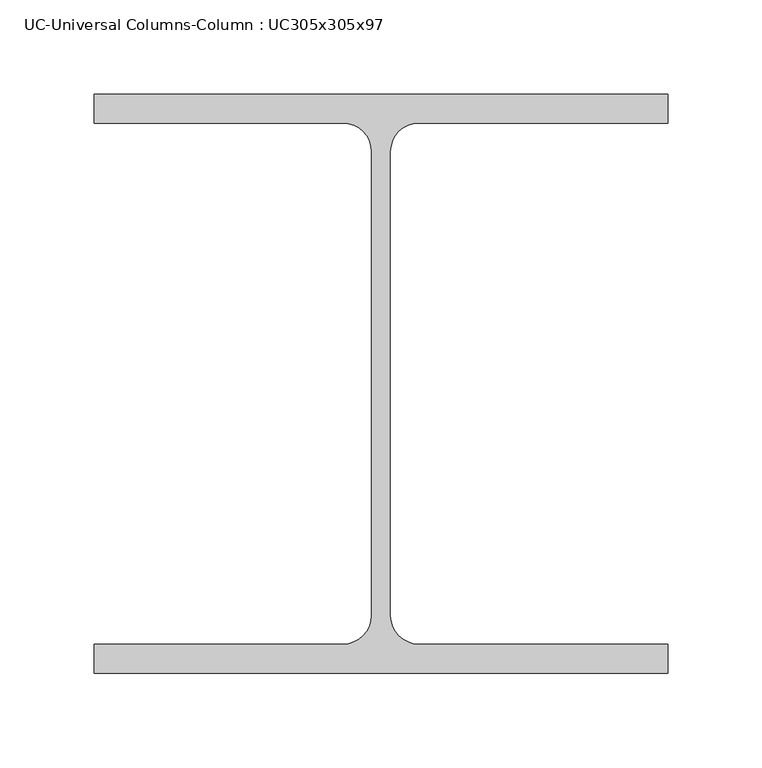
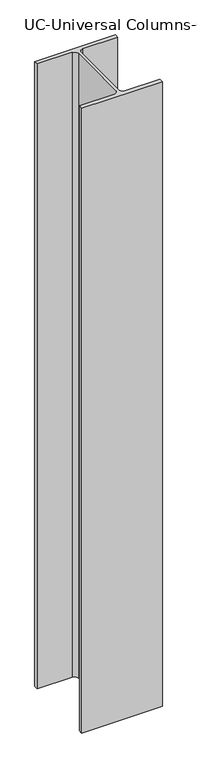
"""IFC4 building model written with IfcOpenShell, lengths in millimetres: column geometry, UC-Universal Columns-Column : UC305x305x97."""

import ifcopenshell
import ifcopenshell.guid

model = None  # the IFC model being written
_history = None  # IfcOwnerHistory: only IFC2X3 demands one
_inside = {}  # id of a spatial element -> (the spatial element, [elements in it])
_under = {}  # id of a project, library or spatial element -> (it, [spatial elements below it])
_declared = {}  # id of a project -> (the project, [libraries it declares])
_typed = {}  # id of a type object -> (the type object, [elements of that type])
_made_of = {}  # id of a material, layer set ... -> (it, [elements and type objects made of it])


def new_model(schema):
    """Start an empty IFC model of exactly this schema.

    Asked for "IFC4X3", IfcOpenShell would pick the latest addendum, in which some entities
    have other attributes; the version numbers below select the first issue.
    IFC2X3 requires an IfcOwnerHistory on every rooted entity: one is made here for all.
    """
    global model, _history
    if schema == "IFC4X3":
        model = ifcopenshell.file(schema_version=(4, 3, 0, 0))
    else:
        model = ifcopenshell.file(schema=schema)
    _inside.clear()
    _under.clear()
    _declared.clear()
    _typed.clear()
    _made_of.clear()
    _history = None
    if model.schema == "IFC2X3":
        org = make("IfcOrganization", Name="unknown")
        user = make(
            "IfcPersonAndOrganization",
            ThePerson=make("IfcPerson", FamilyName="unknown"),
            TheOrganization=org,
        )
        app = make(
            "IfcApplication",
            ApplicationDeveloper=org,
            Version="unknown",
            ApplicationFullName="unknown",
            ApplicationIdentifier="unknown",
        )
        _history = make(
            "IfcOwnerHistory",
            OwningUser=user,
            OwningApplication=app,
            ChangeAction="ADDED",
            CreationDate=0,
        )
    return model


def make(cls, **values):
    """One entity of the class cls with the attributes given. An attribute that is None is left unset."""
    return model.create_entity(
        cls, **{name: value for name, value in values.items() if value is not None}
    )


def rooted(cls, **values):
    """An entity with a GlobalId (a new one), such as an element, a storey or a relation."""
    return make(cls, GlobalId=ifcopenshell.guid.new(), OwnerHistory=_history, **values)


def si_unit(unit_type, name, prefix=None):
    """IfcSIUnit, for example si_unit("LENGTHUNIT", "METRE", prefix="MILLI")."""
    return make("IfcSIUnit", UnitType=unit_type, Prefix=prefix, Name=name)


def assignment(units):
    """IfcUnitAssignment: the units of a project."""
    return None if units is None else make("IfcUnitAssignment", Units=units)


def point(xyz):
    """IfcCartesianPoint."""
    return None if xyz is None else make("IfcCartesianPoint", Coordinates=xyz)


def direction(xyz):
    """IfcDirection."""
    return None if xyz is None else make("IfcDirection", DirectionRatios=xyz)


def frame(location, z_axis=None, x_axis=None):
    """IfcAxis2Placement3D, a coordinate frame: its origin and axes. An axis left out is left unset."""
    return make(
        "IfcAxis2Placement3D",
        Location=point(location),
        Axis=direction(z_axis),
        RefDirection=direction(x_axis),
    )


def frame_2d(location, x_axis=None):
    """IfcAxis2Placement2D, a coordinate frame in the plane: its origin and x axis."""
    return make(
        "IfcAxis2Placement2D", Location=point(location), RefDirection=direction(x_axis)
    )


def origin():
    """The frame at (0, 0, 0) with its axes left unset."""
    return frame((0.0, 0.0, 0.0))


def origin_with_axes():
    """The frame at (0, 0, 0) with the z axis (0, 0, 1) and the x axis (1, 0, 0) written out."""
    return frame((0.0, 0.0, 0.0), z_axis=(0.0, 0.0, 1.0), x_axis=(1.0, 0.0, 0.0))


def place(relative_to, where):
    """IfcLocalPlacement: puts the frame where relative to a parent placement (None: the world)."""
    return make(
        "IfcLocalPlacement", PlacementRelTo=relative_to, RelativePlacement=where
    )


def context(
    kind, dimensions, precision=None, world=None, true_north=None, identifier=None
):
    """IfcGeometricRepresentationContext, for example the 3D "Model" context."""
    return make(
        "IfcGeometricRepresentationContext",
        ContextIdentifier=identifier,
        ContextType=kind,
        CoordinateSpaceDimension=dimensions,
        Precision=precision,
        WorldCoordinateSystem=world,
        TrueNorth=true_north,
    )


def project(units=None, contexts=None):
    """IfcProject with its units and contexts."""
    return rooted(
        "IfcProject",
        Name="project",
        RepresentationContexts=contexts,
        UnitsInContext=assignment(units),
    )


def spatial(cls, under=None, at=None, **own):
    """A site, building, storey or space (cls), placed at a placement, below another one or the project."""
    s = rooted(cls, ObjectPlacement=at, **own)
    if under is not None:
        _under.setdefault(under.id(), (under, []))[1].append(s)
    return s


def polyline(points):
    """IfcPolyline through the points."""
    return make("IfcPolyline", Points=[point(p) for p in points])


def circle_curve(where, radius):
    """IfcCircle in the frame where."""
    return make("IfcCircle", Position=where, Radius=radius)


def trimmed(basis, trim1, trim2, sense, master):
    """IfcTrimmedCurve: the piece of a basis curve between two trims."""
    return make(
        "IfcTrimmedCurve",
        BasisCurve=basis,
        Trim1=trim1,
        Trim2=trim2,
        SenseAgreement=sense,
        MasterRepresentation=master,
    )


def segment(curve, same_sense, transition):
    """IfcCompositeCurveSegment."""
    return make(
        "IfcCompositeCurveSegment",
        Transition=transition,
        SameSense=same_sense,
        ParentCurve=curve,
    )


def composite_curve(segments, self_intersect=None):
    """IfcCompositeCurve: segments joined end to end."""
    return make("IfcCompositeCurve", Segments=segments, SelfIntersect=self_intersect)


def outline(outer, holes=None, kind="AREA"):
    """IfcArbitraryClosedProfileDef: a profile drawn as a closed curve; with holes, ...WithVoids."""
    if holes is None:
        return make("IfcArbitraryClosedProfileDef", ProfileType=kind, OuterCurve=outer)
    return make(
        "IfcArbitraryProfileDefWithVoids",
        ProfileType=kind,
        OuterCurve=outer,
        InnerCurves=holes,
    )


def extrude(swept, where, along, depth):
    """IfcExtrudedAreaSolid: the profile swept, set in the frame where, extruded along a direction by depth."""
    return make(
        "IfcExtrudedAreaSolid",
        SweptArea=swept,
        Position=where,
        ExtrudedDirection=direction(along),
        Depth=depth,
    )


def shape(context_of_items, identifier, shape_type, items):
    """IfcShapeRepresentation: the items that make up one representation, for example the "Body"."""
    return make(
        "IfcShapeRepresentation",
        ContextOfItems=context_of_items,
        RepresentationIdentifier=identifier,
        RepresentationType=shape_type,
        Items=items,
    )


def source(mapping_origin, context_of_items, identifier, shape_type, items):
    """IfcRepresentationMap: a shape defined once, which mapped items show again and again."""
    return make(
        "IfcRepresentationMap",
        MappingOrigin=mapping_origin,
        MappedRepresentation=shape(context_of_items, identifier, shape_type, items),
    )


def transform(
    local_origin,
    x_axis=None,
    y_axis=None,
    z_axis=None,
    scale=None,
    scale2=None,
    scale3=None,
    uniform=True,
):
    """IfcCartesianTransformationOperator3D, or its non-uniform kind. x_axis, y_axis, z_axis: its Axis1, 2, 3."""
    if uniform:
        return make(
            "IfcCartesianTransformationOperator3D",
            Axis1=direction(x_axis),
            Axis2=direction(y_axis),
            LocalOrigin=point(local_origin),
            Scale=scale,
            Axis3=direction(z_axis),
        )
    return make(
        "IfcCartesianTransformationOperator3DnonUniform",
        Axis1=direction(x_axis),
        Axis2=direction(y_axis),
        LocalOrigin=point(local_origin),
        Scale=scale,
        Axis3=direction(z_axis),
        Scale2=scale2,
        Scale3=scale3,
    )


def mapped(mapping_source, mapping_target):
    """IfcMappedItem: shows the shape of a source again, moved by a transform."""
    return make(
        "IfcMappedItem", MappingSource=mapping_source, MappingTarget=mapping_target
    )


def made_of(thing, what):
    """Note that an element or type object is made of a material, layer set ...; save() writes the relation."""
    if what is not None:
        _made_of.setdefault(what.id(), (what, []))[1].append(thing)
    return thing


def element(
    cls,
    number,
    at=None,
    inside=None,
    cuts=None,
    type_object=None,
    material=None,
    context=None,
    identifier="Body",
    shape_type=None,
    held_by="IfcProductDefinitionShape",
    body=None,
    shapes=None,
    **own,
):
    """One element of the class cls, such as IfcWall. Its Tag is "e" and its number.

    at: its placement. inside: the storey or other place that contains it. cuts: it is an
    opening in that element (IfcRelVoidsElement). A single representation is given by context,
    identifier, shape_type and body (its items); several are given by shapes. held_by: the class
    of the entity that holds the representations. save() writes the other relations.
    """
    e = rooted(cls, Tag="e%d" % number, ObjectPlacement=at, **own)
    if body is not None:
        shapes = [shape(context, identifier, shape_type, body)]
    if shapes is not None:
        e.Representation = make(held_by, Representations=shapes)
    if inside is not None:
        _inside.setdefault(inside.id(), (inside, []))[1].append(e)
    if cuts is not None:
        rooted(
            "IfcRelVoidsElement", RelatingBuildingElement=cuts, RelatedOpeningElement=e
        )
    if type_object is not None:
        _typed.setdefault(type_object.id(), (type_object, []))[1].append(e)
    return made_of(e, material)


def aggregate(whole, parts):
    """IfcRelAggregates: a whole, such as a stair, and the parts it consists of."""
    return rooted("IfcRelAggregates", RelatingObject=whole, RelatedObjects=parts)


def save(model, path):
    """Write the relations noted so far, then the file.

    IfcRelAggregates (storeys below a building ...), IfcRelContainedInSpatialStructure (elements
    in a storey), IfcRelDefinesByType, IfcRelAssociatesMaterial and IfcRelDeclares: one each for
    every whole, place, type object, material and project.
    """
    for whole, parts in _under.values():
        aggregate(whole, parts)
    for where, things in _inside.values():
        rooted(
            "IfcRelContainedInSpatialStructure",
            RelatedElements=things,
            RelatingStructure=where,
        )
    for kind, things in _typed.values():
        rooted("IfcRelDefinesByType", RelatedObjects=things, RelatingType=kind)
    for what, things in _made_of.values():
        rooted("IfcRelAssociatesMaterial", RelatedObjects=things, RelatingMaterial=what)
    for by, libraries in _declared.values():
        rooted("IfcRelDeclares", RelatingContext=by, RelatedDefinitions=libraries)
    model.write(path)


def uc_universal_columns_column_uc305x305x97_3ae92ab7(model_context):
    return source(origin(), model_context, "Body", "SweptSolid", [
        extrude(outline(composite_curve([segment(polyline([(152.65, 153.95), (152.65, 138.55), (20.15, 138.55)]), True, "CONTINUOUS"), segment(trimmed(circle_curve(frame_2d((20.15, 123.35)), 15.2), [point((20.15, 138.55))], [point((4.95, 123.35))], True, "CARTESIAN"), True, "CONTINUOUS"), segment(polyline([(4.95, 123.35), (4.95, -123.35)]), True, "CONTINUOUS"), segment(trimmed(circle_curve(frame_2d((20.15, -123.35)), 15.2), [point((4.95, -123.35))], [point((20.15, -138.55))], True, "CARTESIAN"), True, "CONTINUOUS"), segment(polyline([(20.15, -138.55), (152.65, -138.55), (152.65, -153.95), (-152.65, -153.95), (-152.65, -138.55), (-20.15, -138.55)]), True, "CONTINUOUS"), segment(trimmed(circle_curve(frame_2d((-20.15, -123.35)), 15.2), [point((-20.15, -138.55))], [point((-4.95, -123.35))], True, "CARTESIAN"), True, "CONTINUOUS"), segment(polyline([(-4.95, -123.35), (-4.95, 123.35)]), True, "CONTINUOUS"), segment(trimmed(circle_curve(frame_2d((-20.15, 123.35)), 15.2), [point((-4.95, 123.35))], [point((-20.15, 138.55))], True, "CARTESIAN"), True, "CONTINUOUS"), segment(polyline([(-20.15, 138.55), (-152.65, 138.55), (-152.65, 153.95), (152.65, 153.95)]), True, "CONTINUOUS")], self_intersect=False)), origin_with_axes(), (0.0, 0.0, 1.0), 2500.0),
    ])


if __name__ == "__main__":
    model = new_model("IFC4")
    model_context = context("Model", 3, world=origin())
    ifc_project = project(units=[si_unit("LENGTHUNIT", "METRE", prefix="MILLI")], contexts=[model_context])
    site = spatial("IfcSite", under=ifc_project)
    building = spatial("IfcBuilding", under=site)
    placement = place(None, origin())
    uc_universal_columns_column_uc305x305x97_shape = uc_universal_columns_column_uc305x305x97_3ae92ab7(model_context)
    element("IfcColumn", 1, ObjectType="UC-Universal Columns-Column : UC305x305x97", at=placement, inside=building, context=model_context, shape_type="MappedRepresentation", body=[
        mapped(uc_universal_columns_column_uc305x305x97_shape, transform((0.0, 0.0, 0.0), x_axis=(1.0, 0.0, 0.0), y_axis=(0.0, 1.0, 0.0), z_axis=(0.0, 0.0, 1.0))),
    ])
    save(model, "model.ifc")

# Revit data of these elements
# Type "UC-Universal Columns-Column : UC305x305x97"
#   Section Name Key = "UC305x305x97"
#   Width = 30.53 cm
#   Web Thickness = 0.99 cm
#   Web Fillet = 1.52 cm
#   Warping Constant = 1560000.0 cm⁶
#   Torsional Moment of Inertia = 91.20 cm⁴
#   Section Area = 123.0 cm²
#   Plastic Modulus weak axis = 726.0 cm³
#   Plastic Modulus strong axis = 1592.0 cm³
#   Nominal Weight = 96.8996 kgf/m
#   Moment of Inertia weak axis = 7308.00 cm⁴
#   Moment of Inertia strong axis = 22249.00 cm⁴
#   Height = 30.79 cm
#   Flange Thickness = 1.54 cm
#   Elastic Modulus weak axis = 479.0 cm³
#   Elastic Modulus strong axis = 1445.0 cm³
#   Centroid Vertical = 15.395 cm
#   Centroid Horizontal = 15.265 cm
#   Bolt Spacing = 14.0 cm
#   Structural Material [instance default] = Metal - Steel 43-275
#   Type Comments = ""
#   Assembly Code = ""
# Element 1 (IfcColumn, "UC-Universal Columns-Column : UC305x305x97")
#   Materials on its faces: "Metal - Steel 43-275"
# Materials
#   "Metal - Steel 43-275": class "Metal", colour RGB 247 247 247, transparency 0, Cost = 0
